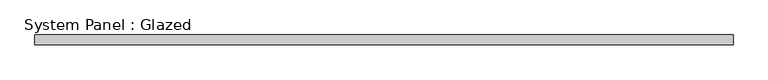
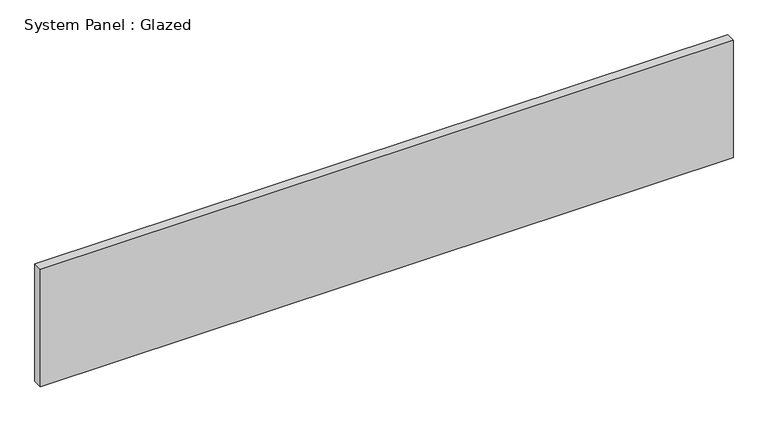
"""IFC4 building model written with IfcOpenShell, lengths in millimetres: plate geometry, System Panel : Glazed."""

from ifc_helpers import new_model, si_unit, origin, origin_with_axes, place, context, project, spatial, polyline, outline, extrude, source, transform, mapped, element, save


def system_panel_glazed_ea680250(model_context):
    return source(origin(), model_context, "Body", "SweptSolid", [
        extrude(outline(polyline([(902.5000002, 24.5), (-902.5000002, 24.5), (-902.5000002, 49.5), (902.5000002, 49.5), (902.5000002, 24.5)])), origin_with_axes(), (0.0, 0.0, 1.0), 323.8777657),
    ])


if __name__ == "__main__":
    model = new_model("IFC4")
    model_context = context("Model", 3, world=origin())
    ifc_project = project(units=[si_unit("LENGTHUNIT", "METRE", prefix="MILLI")], contexts=[model_context])
    site = spatial("IfcSite", under=ifc_project)
    building = spatial("IfcBuilding", under=site)
    placement = place(None, origin())
    system_panel_glazed_shape = system_panel_glazed_ea680250(model_context)
    element("IfcPlate", 1, ObjectType="System Panel : Glazed", at=placement, inside=building, context=model_context, shape_type="MappedRepresentation", body=[
        mapped(system_panel_glazed_shape, transform((0.0, 0.0, 0.0), x_axis=(1.0, 0.0, 0.0), y_axis=(0.0, 1.0, 0.0), z_axis=(0.0, 0.0, 1.0))),
    ])
    save(model, "model.ifc")

# Revit data of these elements
# Element 1 (IfcPlate, "System Panel : Glazed")
#   Materials on its faces: "Glass"
# Materials
#   "Glass": class "Glass", colour RGB 218 227 224, transparency 0.85, Description = "Soda Lime Glass", Cost = 0
